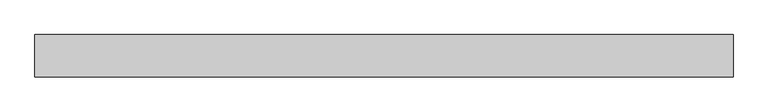
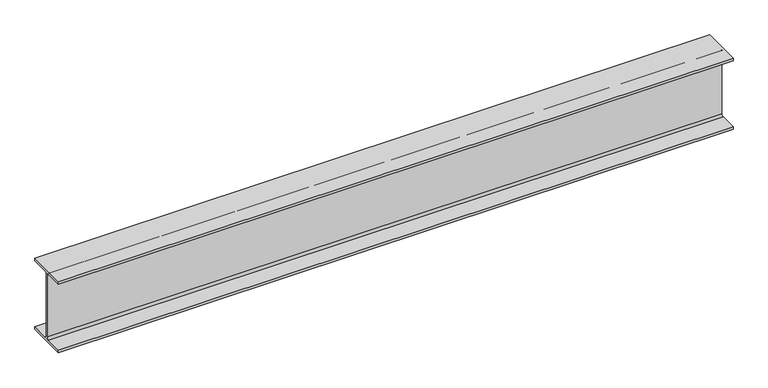
"""IFC4 building model written with IfcOpenShell, lengths in millimetres: beam geometry, Old_Steel Beam_H-KSD3502 : H_SB_ASB_H-194×150x6x9."""

import ifcopenshell
import ifcopenshell.guid

model = None  # the IFC model being written
_history = None  # IfcOwnerHistory: only IFC2X3 demands one
_inside = {}  # id of a spatial element -> (the spatial element, [elements in it])
_under = {}  # id of a project, library or spatial element -> (it, [spatial elements below it])
_declared = {}  # id of a project -> (the project, [libraries it declares])
_typed = {}  # id of a type object -> (the type object, [elements of that type])
_made_of = {}  # id of a material, layer set ... -> (it, [elements and type objects made of it])


def new_model(schema):
    """Start an empty IFC model of exactly this schema.

    Asked for "IFC4X3", IfcOpenShell would pick the latest addendum, in which some entities
    have other attributes; the version numbers below select the first issue.
    IFC2X3 requires an IfcOwnerHistory on every rooted entity: one is made here for all.
    """
    global model, _history
    if schema == "IFC4X3":
        model = ifcopenshell.file(schema_version=(4, 3, 0, 0))
    else:
        model = ifcopenshell.file(schema=schema)
    _inside.clear()
    _under.clear()
    _declared.clear()
    _typed.clear()
    _made_of.clear()
    _history = None
    if model.schema == "IFC2X3":
        org = make("IfcOrganization", Name="unknown")
        user = make(
            "IfcPersonAndOrganization",
            ThePerson=make("IfcPerson", FamilyName="unknown"),
            TheOrganization=org,
        )
        app = make(
            "IfcApplication",
            ApplicationDeveloper=org,
            Version="unknown",
            ApplicationFullName="unknown",
            ApplicationIdentifier="unknown",
        )
        _history = make(
            "IfcOwnerHistory",
            OwningUser=user,
            OwningApplication=app,
            ChangeAction="ADDED",
            CreationDate=0,
        )
    return model


def make(cls, **values):
    """One entity of the class cls with the attributes given. An attribute that is None is left unset."""
    return model.create_entity(
        cls, **{name: value for name, value in values.items() if value is not None}
    )


def rooted(cls, **values):
    """An entity with a GlobalId (a new one), such as an element, a storey or a relation."""
    return make(cls, GlobalId=ifcopenshell.guid.new(), OwnerHistory=_history, **values)


def si_unit(unit_type, name, prefix=None):
    """IfcSIUnit, for example si_unit("LENGTHUNIT", "METRE", prefix="MILLI")."""
    return make("IfcSIUnit", UnitType=unit_type, Prefix=prefix, Name=name)


def assignment(units):
    """IfcUnitAssignment: the units of a project."""
    return None if units is None else make("IfcUnitAssignment", Units=units)


def point(xyz):
    """IfcCartesianPoint."""
    return None if xyz is None else make("IfcCartesianPoint", Coordinates=xyz)


def direction(xyz):
    """IfcDirection."""
    return None if xyz is None else make("IfcDirection", DirectionRatios=xyz)


def frame(location, z_axis=None, x_axis=None):
    """IfcAxis2Placement3D, a coordinate frame: its origin and axes. An axis left out is left unset."""
    return make(
        "IfcAxis2Placement3D",
        Location=point(location),
        Axis=direction(z_axis),
        RefDirection=direction(x_axis),
    )


def frame_2d(location, x_axis=None):
    """IfcAxis2Placement2D, a coordinate frame in the plane: its origin and x axis."""
    return make(
        "IfcAxis2Placement2D", Location=point(location), RefDirection=direction(x_axis)
    )


def origin():
    """The frame at (0, 0, 0) with its axes left unset."""
    return frame((0.0, 0.0, 0.0))


def place(relative_to, where):
    """IfcLocalPlacement: puts the frame where relative to a parent placement (None: the world)."""
    return make(
        "IfcLocalPlacement", PlacementRelTo=relative_to, RelativePlacement=where
    )


def context(
    kind, dimensions, precision=None, world=None, true_north=None, identifier=None
):
    """IfcGeometricRepresentationContext, for example the 3D "Model" context."""
    return make(
        "IfcGeometricRepresentationContext",
        ContextIdentifier=identifier,
        ContextType=kind,
        CoordinateSpaceDimension=dimensions,
        Precision=precision,
        WorldCoordinateSystem=world,
        TrueNorth=true_north,
    )


def project(units=None, contexts=None):
    """IfcProject with its units and contexts."""
    return rooted(
        "IfcProject",
        Name="project",
        RepresentationContexts=contexts,
        UnitsInContext=assignment(units),
    )


def spatial(cls, under=None, at=None, **own):
    """A site, building, storey or space (cls), placed at a placement, below another one or the project."""
    s = rooted(cls, ObjectPlacement=at, **own)
    if under is not None:
        _under.setdefault(under.id(), (under, []))[1].append(s)
    return s


def polyline(points):
    """IfcPolyline through the points."""
    return make("IfcPolyline", Points=[point(p) for p in points])


def circle_curve(where, radius):
    """IfcCircle in the frame where."""
    return make("IfcCircle", Position=where, Radius=radius)


def trimmed(basis, trim1, trim2, sense, master):
    """IfcTrimmedCurve: the piece of a basis curve between two trims."""
    return make(
        "IfcTrimmedCurve",
        BasisCurve=basis,
        Trim1=trim1,
        Trim2=trim2,
        SenseAgreement=sense,
        MasterRepresentation=master,
    )


def segment(curve, same_sense, transition):
    """IfcCompositeCurveSegment."""
    return make(
        "IfcCompositeCurveSegment",
        Transition=transition,
        SameSense=same_sense,
        ParentCurve=curve,
    )


def composite_curve(segments, self_intersect=None):
    """IfcCompositeCurve: segments joined end to end."""
    return make("IfcCompositeCurve", Segments=segments, SelfIntersect=self_intersect)


def outline(outer, holes=None, kind="AREA"):
    """IfcArbitraryClosedProfileDef: a profile drawn as a closed curve; with holes, ...WithVoids."""
    if holes is None:
        return make("IfcArbitraryClosedProfileDef", ProfileType=kind, OuterCurve=outer)
    return make(
        "IfcArbitraryProfileDefWithVoids",
        ProfileType=kind,
        OuterCurve=outer,
        InnerCurves=holes,
    )


def extrude(swept, where, along, depth):
    """IfcExtrudedAreaSolid: the profile swept, set in the frame where, extruded along a direction by depth."""
    return make(
        "IfcExtrudedAreaSolid",
        SweptArea=swept,
        Position=where,
        ExtrudedDirection=direction(along),
        Depth=depth,
    )


def shape(context_of_items, identifier, shape_type, items):
    """IfcShapeRepresentation: the items that make up one representation, for example the "Body"."""
    return make(
        "IfcShapeRepresentation",
        ContextOfItems=context_of_items,
        RepresentationIdentifier=identifier,
        RepresentationType=shape_type,
        Items=items,
    )


def source(mapping_origin, context_of_items, identifier, shape_type, items):
    """IfcRepresentationMap: a shape defined once, which mapped items show again and again."""
    return make(
        "IfcRepresentationMap",
        MappingOrigin=mapping_origin,
        MappedRepresentation=shape(context_of_items, identifier, shape_type, items),
    )


def transform(
    local_origin,
    x_axis=None,
    y_axis=None,
    z_axis=None,
    scale=None,
    scale2=None,
    scale3=None,
    uniform=True,
):
    """IfcCartesianTransformationOperator3D, or its non-uniform kind. x_axis, y_axis, z_axis: its Axis1, 2, 3."""
    if uniform:
        return make(
            "IfcCartesianTransformationOperator3D",
            Axis1=direction(x_axis),
            Axis2=direction(y_axis),
            LocalOrigin=point(local_origin),
            Scale=scale,
            Axis3=direction(z_axis),
        )
    return make(
        "IfcCartesianTransformationOperator3DnonUniform",
        Axis1=direction(x_axis),
        Axis2=direction(y_axis),
        LocalOrigin=point(local_origin),
        Scale=scale,
        Axis3=direction(z_axis),
        Scale2=scale2,
        Scale3=scale3,
    )


def mapped(mapping_source, mapping_target):
    """IfcMappedItem: shows the shape of a source again, moved by a transform."""
    return make(
        "IfcMappedItem", MappingSource=mapping_source, MappingTarget=mapping_target
    )


def made_of(thing, what):
    """Note that an element or type object is made of a material, layer set ...; save() writes the relation."""
    if what is not None:
        _made_of.setdefault(what.id(), (what, []))[1].append(thing)
    return thing


def element(
    cls,
    number,
    at=None,
    inside=None,
    cuts=None,
    type_object=None,
    material=None,
    context=None,
    identifier="Body",
    shape_type=None,
    held_by="IfcProductDefinitionShape",
    body=None,
    shapes=None,
    **own,
):
    """One element of the class cls, such as IfcWall. Its Tag is "e" and its number.

    at: its placement. inside: the storey or other place that contains it. cuts: it is an
    opening in that element (IfcRelVoidsElement). A single representation is given by context,
    identifier, shape_type and body (its items); several are given by shapes. held_by: the class
    of the entity that holds the representations. save() writes the other relations.
    """
    e = rooted(cls, Tag="e%d" % number, ObjectPlacement=at, **own)
    if body is not None:
        shapes = [shape(context, identifier, shape_type, body)]
    if shapes is not None:
        e.Representation = make(held_by, Representations=shapes)
    if inside is not None:
        _inside.setdefault(inside.id(), (inside, []))[1].append(e)
    if cuts is not None:
        rooted(
            "IfcRelVoidsElement", RelatingBuildingElement=cuts, RelatedOpeningElement=e
        )
    if type_object is not None:
        _typed.setdefault(type_object.id(), (type_object, []))[1].append(e)
    return made_of(e, material)


def aggregate(whole, parts):
    """IfcRelAggregates: a whole, such as a stair, and the parts it consists of."""
    return rooted("IfcRelAggregates", RelatingObject=whole, RelatedObjects=parts)


def save(model, path):
    """Write the relations noted so far, then the file.

    IfcRelAggregates (storeys below a building ...), IfcRelContainedInSpatialStructure (elements
    in a storey), IfcRelDefinesByType, IfcRelAssociatesMaterial and IfcRelDeclares: one each for
    every whole, place, type object, material and project.
    """
    for whole, parts in _under.values():
        aggregate(whole, parts)
    for where, things in _inside.values():
        rooted(
            "IfcRelContainedInSpatialStructure",
            RelatedElements=things,
            RelatingStructure=where,
        )
    for kind, things in _typed.values():
        rooted("IfcRelDefinesByType", RelatedObjects=things, RelatingType=kind)
    for what, things in _made_of.values():
        rooted("IfcRelAssociatesMaterial", RelatedObjects=things, RelatingMaterial=what)
    for by, libraries in _declared.values():
        rooted("IfcRelDeclares", RelatingContext=by, RelatedDefinitions=libraries)
    model.write(path)


def beam_157ca0d3(model_context):
    return source(origin(), model_context, "Body", "SweptSolid", [
        extrude(outline(composite_curve([segment(polyline([(82.5, -141.5), (82.5, -151.7), (-82.5, -151.7), (-82.5, -141.5), (-11.9, -141.5)]), True, "CONTINUOUS"), segment(trimmed(circle_curve(frame_2d((-11.9, -132.6)), 8.9), [point((-11.9, -141.5))], [point((-3.0, -132.6))], True, "CARTESIAN"), True, "CONTINUOUS"), segment(polyline([(-3.0, -132.6), (-3.0, 132.6)]), True, "CONTINUOUS"), segment(trimmed(circle_curve(frame_2d((-11.9, 132.6)), 8.9), [point((-3.0, 132.6))], [point((-11.9, 141.5))], True, "CARTESIAN"), True, "CONTINUOUS"), segment(polyline([(-11.9, 141.5), (-82.5, 141.5), (-82.5, 151.7), (82.5, 151.7), (82.5, 141.5), (11.9, 141.5)]), True, "CONTINUOUS"), segment(trimmed(circle_curve(frame_2d((11.9, 132.6)), 8.9), [point((11.9, 141.5))], [point((3.0, 132.6))], True, "CARTESIAN"), True, "CONTINUOUS"), segment(polyline([(3.0, 132.6), (3.0, -132.6)]), True, "CONTINUOUS"), segment(trimmed(circle_curve(frame_2d((11.9, -132.6)), 8.9), [point((3.0, -132.6))], [point((11.9, -141.5))], True, "CARTESIAN"), True, "CONTINUOUS"), segment(polyline([(11.9, -141.5), (82.5, -141.5)]), True, "CONTINUOUS")], self_intersect=False)), frame((-1236.0559406, 0.0, 0.0), z_axis=(1.0, 0.0, 0.0), x_axis=(0.0, 1.0, 0.0)), (0.0, 0.0, 1.0), 2729.2385396),
    ])


if __name__ == "__main__":
    model = new_model("IFC4")
    model_context = context("Model", 3, world=origin())
    ifc_project = project(units=[si_unit("LENGTHUNIT", "METRE", prefix="MILLI")], contexts=[model_context])
    site = spatial("IfcSite", under=ifc_project)
    building = spatial("IfcBuilding", under=site)
    placement = place(None, origin())
    beam_shape = beam_157ca0d3(model_context)
    element("IfcBeam", 1, ObjectType="Old_Steel Beam_H-KSD3502 : H_SB_ASB_H-194×150x6x9", at=placement, inside=building, context=model_context, shape_type="MappedRepresentation", body=[
        mapped(beam_shape, transform((0.0, 0.0, 0.0), x_axis=(1.0, 0.0, 0.0), y_axis=(0.0, 1.0, 0.0), z_axis=(0.0, 0.0, 1.0))),
    ])
    save(model, "model.ifc")

# Revit data of these elements
# Type "Old_Steel Beam_H-KSD3502 : H_SB_ASB_H-194×150x6x9"
#   Width = 15.0 cm
#   Web Thickness = 0.6 cm
#   Web Fillet = 1.3 cm
#   Warping Constant = 43316.0 cm⁶
#   Torsional Moment of Inertia = 8.622 cm⁴
#   Torsional Modulus = 1.0 cm³
#   Section Area = 39.01 cm²
#   Plastic Modulus weak axis = 104.0 cm³
#   Plastic Modulus strong axis = 309.0 cm³
#   Perimeter = 0.95 m²/m
#   Nominal Weight = 30.60 kgf/m
#   Moment of Inertia weak axis = 507.00 cm⁴
#   Moment of Inertia strong axis = 2690.00 cm⁴
#   Height = 19.4 cm
#   Flange Thickness = 0.9 cm
#   Elastic Modulus weak axis = 67.6 cm³
#   Elastic Modulus strong axis = 277.0 cm³
#   Centroid Vertical = 9.7 cm
#   Centroid Horizontal = 7.5 cm
#   Length [instance default] = 1.5240 m
#   Structural Material [instance default] = Steel, 45-345
#   Assembly Code = ""
# Element 1 (IfcBeam, "Old_Steel Beam_H-KSD3502 : H_SB_ASB_H-194×150x6x9")
#   Structural Material = none
# Materials
#   "Steel, 45-345": class "Metal", colour RGB 189 187 185, transparency 0, Description = "Steel 345 MPa", Cost = 0
